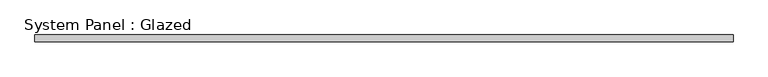
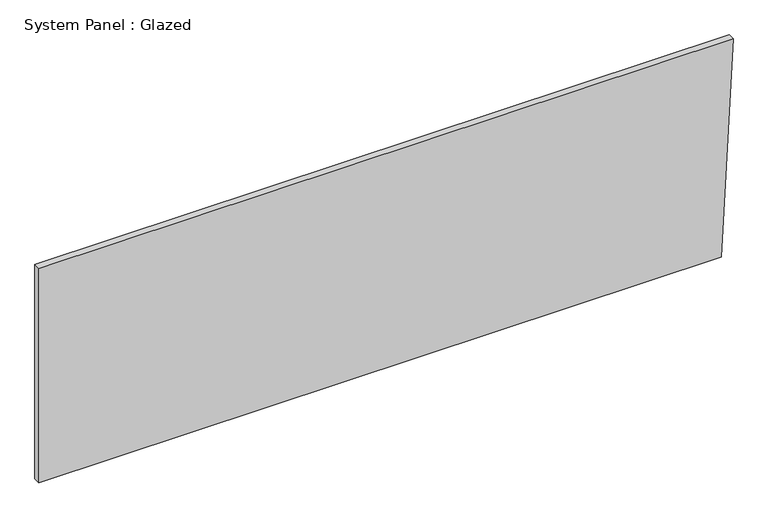
"""IFC4 building model written with IfcOpenShell, lengths in millimetres: plate geometry, System Panel : Glazed."""

from ifc_helpers import new_model, si_unit, frame, origin, place, context, project, spatial, polyline, outline, extrude, source, transform, mapped, element, save


def system_panel_glazed_8e34877b(model_context):
    return source(origin(), model_context, "Body", "SweptSolid", [
        extrude(outline(polyline([(0.0, -1325.8400937), (0.0, 1280.5128872), (866.081558, 1325.8400937), (866.081558, -1325.8400937), (0.0, -1325.8400937)])), frame((0.0, -44.45, 0.0), z_axis=(0.0, 1.0, 0.0), x_axis=(0.0, 0.0, 1.0)), (0.0, 0.0, 1.0), 25.4),
    ])


if __name__ == "__main__":
    model = new_model("IFC4")
    model_context = context("Model", 3, world=origin())
    ifc_project = project(units=[si_unit("LENGTHUNIT", "METRE", prefix="MILLI")], contexts=[model_context])
    site = spatial("IfcSite", under=ifc_project)
    building = spatial("IfcBuilding", under=site)
    placement = place(None, origin())
    system_panel_glazed_shape = system_panel_glazed_8e34877b(model_context)
    element("IfcPlate", 1, ObjectType="System Panel : Glazed", at=placement, inside=building, context=model_context, shape_type="MappedRepresentation", body=[
        mapped(system_panel_glazed_shape, transform((0.0, 0.0, 0.0), x_axis=(1.0, 0.0, 0.0), y_axis=(0.0, 1.0, 0.0), z_axis=(0.0, 0.0, 1.0))),
    ])
    save(model, "model.ifc")

# Revit data of these elements
# Type "System Panel : Glazed"
#   Construction Type Id = "GSP4R"
#   Analytic Construction = "1/8 in Pilkington single glazing"
#   Visual Light Transmittance = 0.9
#   Solar Heat Gain Coefficient = 0.86
#   Heat Transfer Coefficient (U) = 1.18115 BTU/(h·ft²·°F)
#   Define Thermal Properties by = 1
# Element 1 (IfcPlate, "System Panel : Glazed")
#   Materials on its faces: "Glass"
# Materials
#   "Glass": class "Glass", colour RGB 0 128 192, transparency 0.75, Description = "Soda Lime Glass", Cost = 0
